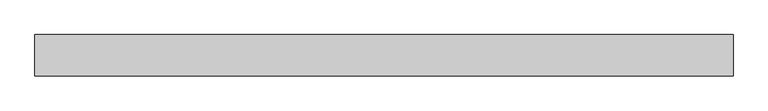
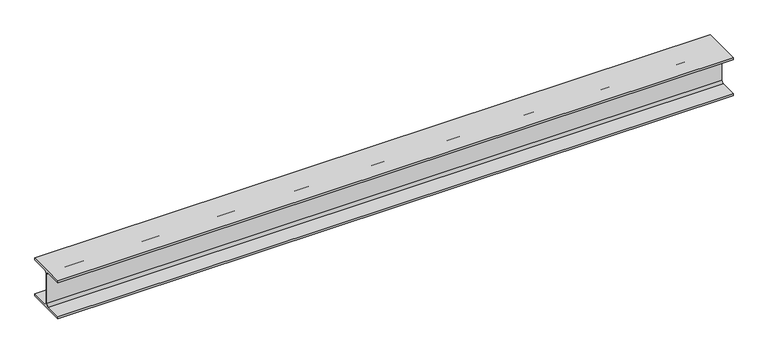
"""IFC4 building model written with IfcOpenShell, lengths in millimetres: beam geometry, 0912_Steel Framing_H-KSD3502 : H_SB_ASB_H-300x300x10x15."""

import ifcopenshell
import ifcopenshell.guid

model = None  # the IFC model being written
_history = None  # IfcOwnerHistory: only IFC2X3 demands one
_inside = {}  # id of a spatial element -> (the spatial element, [elements in it])
_under = {}  # id of a project, library or spatial element -> (it, [spatial elements below it])
_declared = {}  # id of a project -> (the project, [libraries it declares])
_typed = {}  # id of a type object -> (the type object, [elements of that type])
_made_of = {}  # id of a material, layer set ... -> (it, [elements and type objects made of it])


def new_model(schema):
    """Start an empty IFC model of exactly this schema.

    Asked for "IFC4X3", IfcOpenShell would pick the latest addendum, in which some entities
    have other attributes; the version numbers below select the first issue.
    IFC2X3 requires an IfcOwnerHistory on every rooted entity: one is made here for all.
    """
    global model, _history
    if schema == "IFC4X3":
        model = ifcopenshell.file(schema_version=(4, 3, 0, 0))
    else:
        model = ifcopenshell.file(schema=schema)
    _inside.clear()
    _under.clear()
    _declared.clear()
    _typed.clear()
    _made_of.clear()
    _history = None
    if model.schema == "IFC2X3":
        org = make("IfcOrganization", Name="unknown")
        user = make(
            "IfcPersonAndOrganization",
            ThePerson=make("IfcPerson", FamilyName="unknown"),
            TheOrganization=org,
        )
        app = make(
            "IfcApplication",
            ApplicationDeveloper=org,
            Version="unknown",
            ApplicationFullName="unknown",
            ApplicationIdentifier="unknown",
        )
        _history = make(
            "IfcOwnerHistory",
            OwningUser=user,
            OwningApplication=app,
            ChangeAction="ADDED",
            CreationDate=0,
        )
    return model


def make(cls, **values):
    """One entity of the class cls with the attributes given. An attribute that is None is left unset."""
    return model.create_entity(
        cls, **{name: value for name, value in values.items() if value is not None}
    )


def rooted(cls, **values):
    """An entity with a GlobalId (a new one), such as an element, a storey or a relation."""
    return make(cls, GlobalId=ifcopenshell.guid.new(), OwnerHistory=_history, **values)


def si_unit(unit_type, name, prefix=None):
    """IfcSIUnit, for example si_unit("LENGTHUNIT", "METRE", prefix="MILLI")."""
    return make("IfcSIUnit", UnitType=unit_type, Prefix=prefix, Name=name)


def assignment(units):
    """IfcUnitAssignment: the units of a project."""
    return None if units is None else make("IfcUnitAssignment", Units=units)


def point(xyz):
    """IfcCartesianPoint."""
    return None if xyz is None else make("IfcCartesianPoint", Coordinates=xyz)


def direction(xyz):
    """IfcDirection."""
    return None if xyz is None else make("IfcDirection", DirectionRatios=xyz)


def frame(location, z_axis=None, x_axis=None):
    """IfcAxis2Placement3D, a coordinate frame: its origin and axes. An axis left out is left unset."""
    return make(
        "IfcAxis2Placement3D",
        Location=point(location),
        Axis=direction(z_axis),
        RefDirection=direction(x_axis),
    )


def frame_2d(location, x_axis=None):
    """IfcAxis2Placement2D, a coordinate frame in the plane: its origin and x axis."""
    return make(
        "IfcAxis2Placement2D", Location=point(location), RefDirection=direction(x_axis)
    )


def origin():
    """The frame at (0, 0, 0) with its axes left unset."""
    return frame((0.0, 0.0, 0.0))


def place(relative_to, where):
    """IfcLocalPlacement: puts the frame where relative to a parent placement (None: the world)."""
    return make(
        "IfcLocalPlacement", PlacementRelTo=relative_to, RelativePlacement=where
    )


def context(
    kind, dimensions, precision=None, world=None, true_north=None, identifier=None
):
    """IfcGeometricRepresentationContext, for example the 3D "Model" context."""
    return make(
        "IfcGeometricRepresentationContext",
        ContextIdentifier=identifier,
        ContextType=kind,
        CoordinateSpaceDimension=dimensions,
        Precision=precision,
        WorldCoordinateSystem=world,
        TrueNorth=true_north,
    )


def project(units=None, contexts=None):
    """IfcProject with its units and contexts."""
    return rooted(
        "IfcProject",
        Name="project",
        RepresentationContexts=contexts,
        UnitsInContext=assignment(units),
    )


def spatial(cls, under=None, at=None, **own):
    """A site, building, storey or space (cls), placed at a placement, below another one or the project."""
    s = rooted(cls, ObjectPlacement=at, **own)
    if under is not None:
        _under.setdefault(under.id(), (under, []))[1].append(s)
    return s


def polyline(points):
    """IfcPolyline through the points."""
    return make("IfcPolyline", Points=[point(p) for p in points])


def circle_curve(where, radius):
    """IfcCircle in the frame where."""
    return make("IfcCircle", Position=where, Radius=radius)


def trimmed(basis, trim1, trim2, sense, master):
    """IfcTrimmedCurve: the piece of a basis curve between two trims."""
    return make(
        "IfcTrimmedCurve",
        BasisCurve=basis,
        Trim1=trim1,
        Trim2=trim2,
        SenseAgreement=sense,
        MasterRepresentation=master,
    )


def segment(curve, same_sense, transition):
    """IfcCompositeCurveSegment."""
    return make(
        "IfcCompositeCurveSegment",
        Transition=transition,
        SameSense=same_sense,
        ParentCurve=curve,
    )


def composite_curve(segments, self_intersect=None):
    """IfcCompositeCurve: segments joined end to end."""
    return make("IfcCompositeCurve", Segments=segments, SelfIntersect=self_intersect)


def outline(outer, holes=None, kind="AREA"):
    """IfcArbitraryClosedProfileDef: a profile drawn as a closed curve; with holes, ...WithVoids."""
    if holes is None:
        return make("IfcArbitraryClosedProfileDef", ProfileType=kind, OuterCurve=outer)
    return make(
        "IfcArbitraryProfileDefWithVoids",
        ProfileType=kind,
        OuterCurve=outer,
        InnerCurves=holes,
    )


def extrude(swept, where, along, depth):
    """IfcExtrudedAreaSolid: the profile swept, set in the frame where, extruded along a direction by depth."""
    return make(
        "IfcExtrudedAreaSolid",
        SweptArea=swept,
        Position=where,
        ExtrudedDirection=direction(along),
        Depth=depth,
    )


def shape(context_of_items, identifier, shape_type, items):
    """IfcShapeRepresentation: the items that make up one representation, for example the "Body"."""
    return make(
        "IfcShapeRepresentation",
        ContextOfItems=context_of_items,
        RepresentationIdentifier=identifier,
        RepresentationType=shape_type,
        Items=items,
    )


def source(mapping_origin, context_of_items, identifier, shape_type, items):
    """IfcRepresentationMap: a shape defined once, which mapped items show again and again."""
    return make(
        "IfcRepresentationMap",
        MappingOrigin=mapping_origin,
        MappedRepresentation=shape(context_of_items, identifier, shape_type, items),
    )


def transform(
    local_origin,
    x_axis=None,
    y_axis=None,
    z_axis=None,
    scale=None,
    scale2=None,
    scale3=None,
    uniform=True,
):
    """IfcCartesianTransformationOperator3D, or its non-uniform kind. x_axis, y_axis, z_axis: its Axis1, 2, 3."""
    if uniform:
        return make(
            "IfcCartesianTransformationOperator3D",
            Axis1=direction(x_axis),
            Axis2=direction(y_axis),
            LocalOrigin=point(local_origin),
            Scale=scale,
            Axis3=direction(z_axis),
        )
    return make(
        "IfcCartesianTransformationOperator3DnonUniform",
        Axis1=direction(x_axis),
        Axis2=direction(y_axis),
        LocalOrigin=point(local_origin),
        Scale=scale,
        Axis3=direction(z_axis),
        Scale2=scale2,
        Scale3=scale3,
    )


def mapped(mapping_source, mapping_target):
    """IfcMappedItem: shows the shape of a source again, moved by a transform."""
    return make(
        "IfcMappedItem", MappingSource=mapping_source, MappingTarget=mapping_target
    )


def made_of(thing, what):
    """Note that an element or type object is made of a material, layer set ...; save() writes the relation."""
    if what is not None:
        _made_of.setdefault(what.id(), (what, []))[1].append(thing)
    return thing


def element(
    cls,
    number,
    at=None,
    inside=None,
    cuts=None,
    type_object=None,
    material=None,
    context=None,
    identifier="Body",
    shape_type=None,
    held_by="IfcProductDefinitionShape",
    body=None,
    shapes=None,
    **own,
):
    """One element of the class cls, such as IfcWall. Its Tag is "e" and its number.

    at: its placement. inside: the storey or other place that contains it. cuts: it is an
    opening in that element (IfcRelVoidsElement). A single representation is given by context,
    identifier, shape_type and body (its items); several are given by shapes. held_by: the class
    of the entity that holds the representations. save() writes the other relations.
    """
    e = rooted(cls, Tag="e%d" % number, ObjectPlacement=at, **own)
    if body is not None:
        shapes = [shape(context, identifier, shape_type, body)]
    if shapes is not None:
        e.Representation = make(held_by, Representations=shapes)
    if inside is not None:
        _inside.setdefault(inside.id(), (inside, []))[1].append(e)
    if cuts is not None:
        rooted(
            "IfcRelVoidsElement", RelatingBuildingElement=cuts, RelatedOpeningElement=e
        )
    if type_object is not None:
        _typed.setdefault(type_object.id(), (type_object, []))[1].append(e)
    return made_of(e, material)


def aggregate(whole, parts):
    """IfcRelAggregates: a whole, such as a stair, and the parts it consists of."""
    return rooted("IfcRelAggregates", RelatingObject=whole, RelatedObjects=parts)


def save(model, path):
    """Write the relations noted so far, then the file.

    IfcRelAggregates (storeys below a building ...), IfcRelContainedInSpatialStructure (elements
    in a storey), IfcRelDefinesByType, IfcRelAssociatesMaterial and IfcRelDeclares: one each for
    every whole, place, type object, material and project.
    """
    for whole, parts in _under.values():
        aggregate(whole, parts)
    for where, things in _inside.values():
        rooted(
            "IfcRelContainedInSpatialStructure",
            RelatedElements=things,
            RelatingStructure=where,
        )
    for kind, things in _typed.values():
        rooted("IfcRelDefinesByType", RelatedObjects=things, RelatingType=kind)
    for what, things in _made_of.values():
        rooted("IfcRelAssociatesMaterial", RelatedObjects=things, RelatingMaterial=what)
    for by, libraries in _declared.values():
        rooted("IfcRelDeclares", RelatingContext=by, RelatedDefinitions=libraries)
    model.write(path)


def beam_61bab96b(model_context):
    return source(origin(), model_context, "Body", "SweptSolid", [
        extrude(outline(composite_curve([segment(polyline([(150.0, -135.0), (150.0, -150.0), (-150.0, -150.0), (-150.0, -135.0), (-23.0, -135.0)]), True, "CONTINUOUS"), segment(trimmed(circle_curve(frame_2d((-23.0, -117.0)), 18.0), [point((-23.0, -135.0))], [point((-5.0, -117.0))], True, "CARTESIAN"), True, "CONTINUOUS"), segment(polyline([(-5.0, -117.0), (-5.0, 117.0)]), True, "CONTINUOUS"), segment(trimmed(circle_curve(frame_2d((-23.0, 117.0)), 18.0), [point((-5.0, 117.0))], [point((-23.0, 135.0))], True, "CARTESIAN"), True, "CONTINUOUS"), segment(polyline([(-23.0, 135.0), (-150.0, 135.0), (-150.0, 150.0), (150.0, 150.0), (150.0, 135.0), (23.0, 135.0)]), True, "CONTINUOUS"), segment(trimmed(circle_curve(frame_2d((23.0, 117.0)), 18.0), [point((23.0, 135.0))], [point((5.0, 117.0))], True, "CARTESIAN"), True, "CONTINUOUS"), segment(polyline([(5.0, 117.0), (5.0, -117.0)]), True, "CONTINUOUS"), segment(trimmed(circle_curve(frame_2d((23.0, -117.0)), 18.0), [point((5.0, -117.0))], [point((23.0, -135.0))], True, "CARTESIAN"), True, "CONTINUOUS"), segment(polyline([(23.0, -135.0), (150.0, -135.0)]), True, "CONTINUOUS")], self_intersect=False)), frame((-2413.6981883, 0.0, 0.0), z_axis=(1.0, 0.0, 0.0), x_axis=(0.0, 1.0, 0.0)), (0.0, 0.0, 1.0), 5076.9152279),
    ])


if __name__ == "__main__":
    model = new_model("IFC4")
    model_context = context("Model", 3, world=origin())
    ifc_project = project(units=[si_unit("LENGTHUNIT", "METRE", prefix="MILLI")], contexts=[model_context])
    site = spatial("IfcSite", under=ifc_project)
    building = spatial("IfcBuilding", under=site)
    placement = place(None, origin())
    beam_shape = beam_61bab96b(model_context)
    element("IfcBeam", 1, ObjectType="0912_Steel Framing_H-KSD3502 : H_SB_ASB_H-300x300x10x15", at=placement, inside=building, context=model_context, shape_type="MappedRepresentation", body=[
        mapped(beam_shape, transform((0.0, 0.0, 0.0), x_axis=(1.0, 0.0, 0.0), y_axis=(0.0, 1.0, 0.0), z_axis=(0.0, 0.0, 1.0))),
    ])
    save(model, "model.ifc")

# Revit data of these elements
# Type "0912_Steel Framing_H-KSD3502 : H_SB_ASB_H-300x300x10x15"
#   H_WM Code_1 = "S01AA001-00001 | Main Steel Structure Fabrication Work | Shelter/Building | Heavy Steel - Standard (Weight≥90KG/M) | Material: (   )"
#   H_WM Code_2 = "S03AA027-00001 | Main Steel Structure Erection Work | Shelter/Building | Heavy Steel (Weight≥90KG/M) | Material: (   )"
#   H_WM Code_3 = "S01AA010-00001 | Main Steel Structure Fabrication Work | Shelter/Building | Steel Painting/Coating | for Non-Fireproofed Steel Surface, Surface Preparation, Primer, Second & Final Coat | Material: (   )"
#   H_Q'ty Cal Type Tag = "SB-Q2"
#   Width = 30.0 cm
#   Web Thickness = 1.0 cm
#   Web Fillet = 1.8 cm
#   Warping Constant = 1370000.0 cm⁶
#   W = 0
#   Torsional Moment of Inertia = 77.00 cm⁴
#   Section Area = 119.8 cm²
#   Plastic Modulus weak axis = 684.0 cm³
#   Plastic Modulus strong axis = 1500.0 cm³
#   Perimeter = 1.75 m²/m
#   Nominal Weight = 94.00 kgf/m
#   Moment of Inertia weak axis = 6750.00 cm⁴
#   Moment of Inertia strong axis = 20400.00 cm⁴
#   Height = 30.0 cm
#   Flange Thickness = 1.5 cm
#   Elastic Modulus weak axis = 450.0 cm³
#   Elastic Modulus strong axis = 1360.0 cm³
#   Centroid Vertical = 15.0 cm
#   Centroid Horizontal = 15.0 cm
#   Ix = 204000000
#   Length [instance default] = 1.5240 m
#   Zx = 1500000
#   b = 0.3000 m
#   h = 0.3000 m
#   r = 0.0180 m
#   s = 0.0100 m
#   t = 0.0150 m
#   A = 0.01198 m²
#   Structural Material [instance default] = Steel, 45-345
#   Assembly Code = ""
# Element 1 (IfcBeam, "0912_Steel Framing_H-KSD3502 : H_SB_ASB_H-300x300x10x15")
#   Structural Material = none
# Materials
#   "Steel, 45-345": class "Metal", colour RGB 189 187 185, transparency 0, Description = "Steel 345 MPa", Cost = 0
